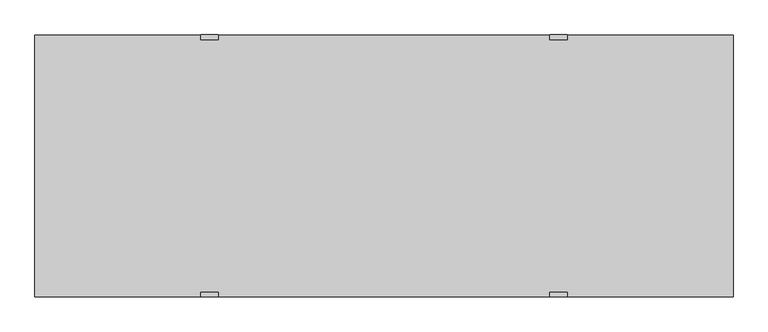
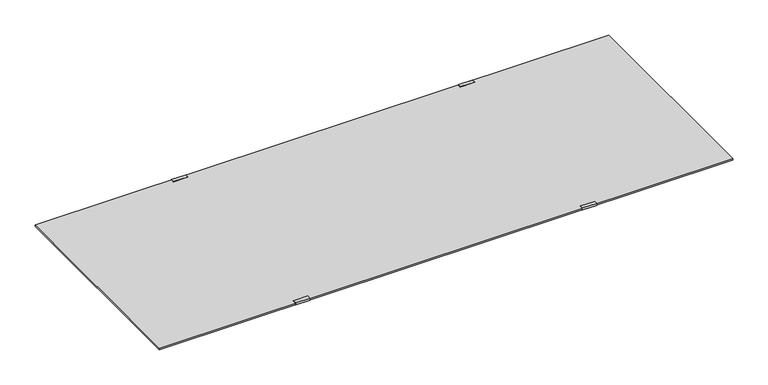
"""IFC4 building model written with IfcOpenShell, lengths in millimetres: proxy geometry."""

from ifc_helpers import new_model, si_unit, frame, origin, origin_with_axes, place, context, project, spatial, polyline, outline, extrude, source, transform, mapped, element, save


def specialty_equipment_fd5685f8(model_context):
    return source(origin(), model_context, "Body", "SweptSolid", [
        extrude(outline(polyline([(-381.0, 6.35), (-381.0, 0.0), (-381.79375, 0.0), (-381.79375, 7.14375), (-368.3, 7.14375), (-368.3, 6.35), (-381.0, 6.35)])), frame((482.6, 0.0, 0.0), z_axis=(1.0, 0.0, 0.0), x_axis=(0.0, 1.0, 0.0)), (0.0, 0.0, 1.0), 50.8),
        extrude(outline(polyline([(-381.0, 6.35), (-381.0, 0.0), (-381.79375, 0.0), (-381.79375, 7.14375), (-368.3, 7.14375), (-368.3, 6.35), (-381.0, 6.35)])), frame((-533.4, 0.0, 0.0), z_axis=(1.0, 0.0, 0.0), x_axis=(0.0, 1.0, 0.0)), (0.0, 0.0, 1.0), 50.8),
        extrude(outline(polyline([(381.0, 6.35), (368.3, 6.35), (368.3, 7.14375), (381.79375, 7.14375), (381.79375, 0.0), (381.0, 0.0), (381.0, 6.35)])), frame((482.6, 0.0, 0.0), z_axis=(1.0, 0.0, 0.0), x_axis=(0.0, 1.0, 0.0)), (0.0, 0.0, 1.0), 50.8),
        extrude(outline(polyline([(381.0, 6.35), (368.3, 6.35), (368.3, 7.14375), (381.79375, 7.14375), (381.79375, 0.0), (381.0, 0.0), (381.0, 6.35)])), frame((-533.4, 0.0, 0.0), z_axis=(1.0, 0.0, 0.0), x_axis=(0.0, 1.0, 0.0)), (0.0, 0.0, 1.0), 50.8),
        extrude(outline(polyline([(1016.0, 381.0), (1016.0, -381.0), (-1016.0, -381.0), (-1016.0, 381.0), (1016.0, 381.0)])), origin_with_axes(), (0.0, 0.0, 1.0), 6.35),
    ])


if __name__ == "__main__":
    model = new_model("IFC4")
    model_context = context("Model", 3, world=origin())
    ifc_project = project(units=[si_unit("LENGTHUNIT", "METRE", prefix="MILLI")], contexts=[model_context])
    site = spatial("IfcSite", under=ifc_project)
    building = spatial("IfcBuilding", under=site)
    placement = place(None, origin())
    specialty_equipment_shape = specialty_equipment_fd5685f8(model_context)
    element("IfcBuildingElementProxy", 1, Name="Bradley-Washroom_Accessories-Mirrors-747_Standard : 60\" x 36\" + BradEX", ObjectType="Bradley-Washroom_Accessories-Mirrors-747_Standard : 60\" x 36\" + BradEX", at=placement, inside=building, context=model_context, shape_type="MappedRepresentation", body=[
        mapped(specialty_equipment_shape, transform((0.0, 0.0, 0.0), x_axis=(1.0, 0.0, 0.0), y_axis=(0.0, 1.0, 0.0), z_axis=(0.0, 0.0, 1.0))),
    ])
    save(model, "model.ifc")

# Revit data of these elements
# Type "Bradley-Washroom_Accessories-Mirrors-747_Standard : 60\" x 36\" + BradEX"
#   Warranty Information = "Complete unit, excepting mirrors warranted for one year.\r\n Stainless steel mirror frames for fifteen years.\r\n Plate glass mirrors for fifteen years.\r\n This warranty does not cover installation or any other labor charges and does not apply to any units,\r\n which have been damaged by accident, abuse, improper installation, improper maintenance, or altered in any way."
#   Version = "1.0"
#   URL = "http://www.bradleycorp.com/"
#   Type Comments = "BradEX 1/4\" Float Glass Mirror"
#   OmniClass Title = "Mirrors"
#   OmniClass Code = "23.40.95.17.17"
#   Modeling Code = ""
#   Model = "747-024360"
#   MasterFormat Title = "Commercial Toilet Accessories"
#   MasterFormat Number = "10 28 13. 13"
#   Manufacturer = "Bradley Corporation"
#   Industry Standards = "ASTM C 1036"
#   Fire Rating = "n/a"
#   Description = "Frameless Mirror, Clip Fasteners, 24 by 36 inches"
#   Copyright = "This Model Data is Property of Bradley Corporation"
#   Buy American Act = "Yes"
#   Assembly Code = "C1030900"
#   ADA Compliant = "Yes"
#   Width = 6' - 8"
#   Height = 2' - 6"
#   Fastener Placement = 1' - 8"
#   Depth = 0' - 0 1/4"
#   Default Elevation = 3' - 4"
#   Reflective Material = Glass - Bradley Corp - BradEX - Polished Float Mirror
#   Frame Material = Bradley Corp Stainless Steel - Satin
# Element 1 (IfcBuildingElementProxy, "Bradley-Washroom_Accessories-Mirrors-747_Standard : 60\" x 36\" + BradEX")
#   Materials on its faces: "Bradley Corp Stainless Steel - Satin", "Glass - Bradley Corp - BradEX - Polished Float Mirror"
# Materials
#   "Glass - Bradley Corp - BradEX - Polished Float Mirror": class "Glass", colour RGB 220 232 220, transparency 0, Manufacturer = "Bradley Corporation", URL = "www.bradleycorp.com", Description = "Stainless Steel - Satin Finish", Cost = 0
#   "Bradley Corp Stainless Steel - Satin": class "Metal", colour RGB 189 187 185, transparency 0, Manufacturer = "Bradley Corporation", URL = "www.bradleycorp.com", Description = "Stainless Steel - Satin Finish", Cost = 0
